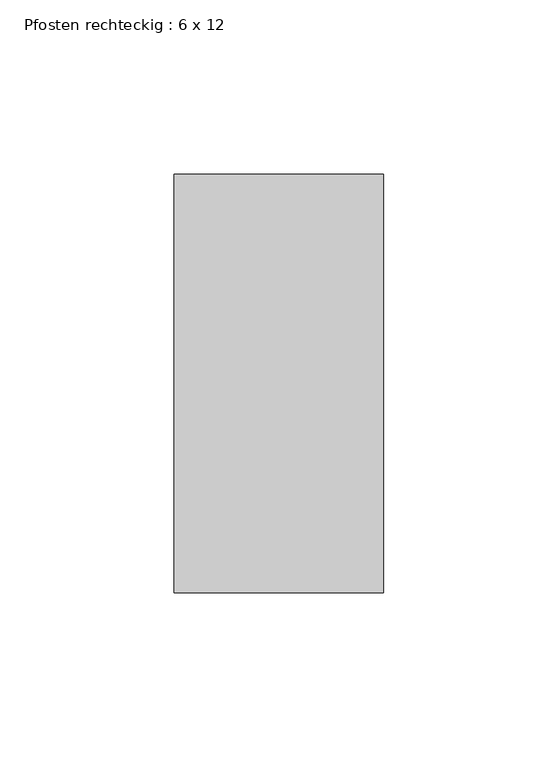
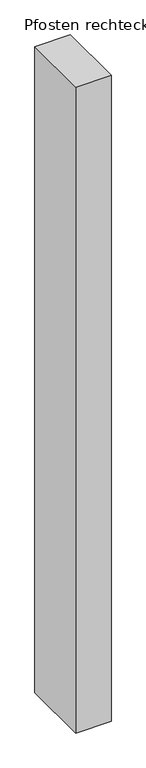
"""IFC4 building model written with IfcOpenShell, lengths in millimetres: member geometry, Pfosten rechteckig : 6 x 12."""

import ifcopenshell
import ifcopenshell.guid

model = None  # the IFC model being written
_history = None  # IfcOwnerHistory: only IFC2X3 demands one
_inside = {}  # id of a spatial element -> (the spatial element, [elements in it])
_under = {}  # id of a project, library or spatial element -> (it, [spatial elements below it])
_declared = {}  # id of a project -> (the project, [libraries it declares])
_typed = {}  # id of a type object -> (the type object, [elements of that type])
_made_of = {}  # id of a material, layer set ... -> (it, [elements and type objects made of it])


def new_model(schema):
    """Start an empty IFC model of exactly this schema.

    Asked for "IFC4X3", IfcOpenShell would pick the latest addendum, in which some entities
    have other attributes; the version numbers below select the first issue.
    IFC2X3 requires an IfcOwnerHistory on every rooted entity: one is made here for all.
    """
    global model, _history
    if schema == "IFC4X3":
        model = ifcopenshell.file(schema_version=(4, 3, 0, 0))
    else:
        model = ifcopenshell.file(schema=schema)
    _inside.clear()
    _under.clear()
    _declared.clear()
    _typed.clear()
    _made_of.clear()
    _history = None
    if model.schema == "IFC2X3":
        org = make("IfcOrganization", Name="unknown")
        user = make(
            "IfcPersonAndOrganization",
            ThePerson=make("IfcPerson", FamilyName="unknown"),
            TheOrganization=org,
        )
        app = make(
            "IfcApplication",
            ApplicationDeveloper=org,
            Version="unknown",
            ApplicationFullName="unknown",
            ApplicationIdentifier="unknown",
        )
        _history = make(
            "IfcOwnerHistory",
            OwningUser=user,
            OwningApplication=app,
            ChangeAction="ADDED",
            CreationDate=0,
        )
    return model


def make(cls, **values):
    """One entity of the class cls with the attributes given. An attribute that is None is left unset."""
    return model.create_entity(
        cls, **{name: value for name, value in values.items() if value is not None}
    )


def rooted(cls, **values):
    """An entity with a GlobalId (a new one), such as an element, a storey or a relation."""
    return make(cls, GlobalId=ifcopenshell.guid.new(), OwnerHistory=_history, **values)


def si_unit(unit_type, name, prefix=None):
    """IfcSIUnit, for example si_unit("LENGTHUNIT", "METRE", prefix="MILLI")."""
    return make("IfcSIUnit", UnitType=unit_type, Prefix=prefix, Name=name)


def assignment(units):
    """IfcUnitAssignment: the units of a project."""
    return None if units is None else make("IfcUnitAssignment", Units=units)


def point(xyz):
    """IfcCartesianPoint."""
    return None if xyz is None else make("IfcCartesianPoint", Coordinates=xyz)


def direction(xyz):
    """IfcDirection."""
    return None if xyz is None else make("IfcDirection", DirectionRatios=xyz)


def frame(location, z_axis=None, x_axis=None):
    """IfcAxis2Placement3D, a coordinate frame: its origin and axes. An axis left out is left unset."""
    return make(
        "IfcAxis2Placement3D",
        Location=point(location),
        Axis=direction(z_axis),
        RefDirection=direction(x_axis),
    )


def origin():
    """The frame at (0, 0, 0) with its axes left unset."""
    return frame((0.0, 0.0, 0.0))


def place(relative_to, where):
    """IfcLocalPlacement: puts the frame where relative to a parent placement (None: the world)."""
    return make(
        "IfcLocalPlacement", PlacementRelTo=relative_to, RelativePlacement=where
    )


def context(
    kind, dimensions, precision=None, world=None, true_north=None, identifier=None
):
    """IfcGeometricRepresentationContext, for example the 3D "Model" context."""
    return make(
        "IfcGeometricRepresentationContext",
        ContextIdentifier=identifier,
        ContextType=kind,
        CoordinateSpaceDimension=dimensions,
        Precision=precision,
        WorldCoordinateSystem=world,
        TrueNorth=true_north,
    )


def project(units=None, contexts=None):
    """IfcProject with its units and contexts."""
    return rooted(
        "IfcProject",
        Name="project",
        RepresentationContexts=contexts,
        UnitsInContext=assignment(units),
    )


def spatial(cls, under=None, at=None, **own):
    """A site, building, storey or space (cls), placed at a placement, below another one or the project."""
    s = rooted(cls, ObjectPlacement=at, **own)
    if under is not None:
        _under.setdefault(under.id(), (under, []))[1].append(s)
    return s


def polyline(points):
    """IfcPolyline through the points."""
    return make("IfcPolyline", Points=[point(p) for p in points])


def outline(outer, holes=None, kind="AREA"):
    """IfcArbitraryClosedProfileDef: a profile drawn as a closed curve; with holes, ...WithVoids."""
    if holes is None:
        return make("IfcArbitraryClosedProfileDef", ProfileType=kind, OuterCurve=outer)
    return make(
        "IfcArbitraryProfileDefWithVoids",
        ProfileType=kind,
        OuterCurve=outer,
        InnerCurves=holes,
    )


def extrude(swept, where, along, depth):
    """IfcExtrudedAreaSolid: the profile swept, set in the frame where, extruded along a direction by depth."""
    return make(
        "IfcExtrudedAreaSolid",
        SweptArea=swept,
        Position=where,
        ExtrudedDirection=direction(along),
        Depth=depth,
    )


def shape(context_of_items, identifier, shape_type, items):
    """IfcShapeRepresentation: the items that make up one representation, for example the "Body"."""
    return make(
        "IfcShapeRepresentation",
        ContextOfItems=context_of_items,
        RepresentationIdentifier=identifier,
        RepresentationType=shape_type,
        Items=items,
    )


def source(mapping_origin, context_of_items, identifier, shape_type, items):
    """IfcRepresentationMap: a shape defined once, which mapped items show again and again."""
    return make(
        "IfcRepresentationMap",
        MappingOrigin=mapping_origin,
        MappedRepresentation=shape(context_of_items, identifier, shape_type, items),
    )


def transform(
    local_origin,
    x_axis=None,
    y_axis=None,
    z_axis=None,
    scale=None,
    scale2=None,
    scale3=None,
    uniform=True,
):
    """IfcCartesianTransformationOperator3D, or its non-uniform kind. x_axis, y_axis, z_axis: its Axis1, 2, 3."""
    if uniform:
        return make(
            "IfcCartesianTransformationOperator3D",
            Axis1=direction(x_axis),
            Axis2=direction(y_axis),
            LocalOrigin=point(local_origin),
            Scale=scale,
            Axis3=direction(z_axis),
        )
    return make(
        "IfcCartesianTransformationOperator3DnonUniform",
        Axis1=direction(x_axis),
        Axis2=direction(y_axis),
        LocalOrigin=point(local_origin),
        Scale=scale,
        Axis3=direction(z_axis),
        Scale2=scale2,
        Scale3=scale3,
    )


def mapped(mapping_source, mapping_target):
    """IfcMappedItem: shows the shape of a source again, moved by a transform."""
    return make(
        "IfcMappedItem", MappingSource=mapping_source, MappingTarget=mapping_target
    )


def made_of(thing, what):
    """Note that an element or type object is made of a material, layer set ...; save() writes the relation."""
    if what is not None:
        _made_of.setdefault(what.id(), (what, []))[1].append(thing)
    return thing


def element(
    cls,
    number,
    at=None,
    inside=None,
    cuts=None,
    type_object=None,
    material=None,
    context=None,
    identifier="Body",
    shape_type=None,
    held_by="IfcProductDefinitionShape",
    body=None,
    shapes=None,
    **own,
):
    """One element of the class cls, such as IfcWall. Its Tag is "e" and its number.

    at: its placement. inside: the storey or other place that contains it. cuts: it is an
    opening in that element (IfcRelVoidsElement). A single representation is given by context,
    identifier, shape_type and body (its items); several are given by shapes. held_by: the class
    of the entity that holds the representations. save() writes the other relations.
    """
    e = rooted(cls, Tag="e%d" % number, ObjectPlacement=at, **own)
    if body is not None:
        shapes = [shape(context, identifier, shape_type, body)]
    if shapes is not None:
        e.Representation = make(held_by, Representations=shapes)
    if inside is not None:
        _inside.setdefault(inside.id(), (inside, []))[1].append(e)
    if cuts is not None:
        rooted(
            "IfcRelVoidsElement", RelatingBuildingElement=cuts, RelatedOpeningElement=e
        )
    if type_object is not None:
        _typed.setdefault(type_object.id(), (type_object, []))[1].append(e)
    return made_of(e, material)


def aggregate(whole, parts):
    """IfcRelAggregates: a whole, such as a stair, and the parts it consists of."""
    return rooted("IfcRelAggregates", RelatingObject=whole, RelatedObjects=parts)


def save(model, path):
    """Write the relations noted so far, then the file.

    IfcRelAggregates (storeys below a building ...), IfcRelContainedInSpatialStructure (elements
    in a storey), IfcRelDefinesByType, IfcRelAssociatesMaterial and IfcRelDeclares: one each for
    every whole, place, type object, material and project.
    """
    for whole, parts in _under.values():
        aggregate(whole, parts)
    for where, things in _inside.values():
        rooted(
            "IfcRelContainedInSpatialStructure",
            RelatedElements=things,
            RelatingStructure=where,
        )
    for kind, things in _typed.values():
        rooted("IfcRelDefinesByType", RelatedObjects=things, RelatingType=kind)
    for what, things in _made_of.values():
        rooted("IfcRelAssociatesMaterial", RelatedObjects=things, RelatingMaterial=what)
    for by, libraries in _declared.values():
        rooted("IfcRelDeclares", RelatingContext=by, RelatedDefinitions=libraries)
    model.write(path)


def pfosten_rechteckig_6_x_12_ce3c1f4b(model_context):
    return source(origin(), model_context, "Body", "SweptSolid", [
        extrude(outline(polyline([(30.0, 60.0), (30.0, -60.0), (-30.0, -60.0), (-30.0, 60.0), (30.0, 60.0)])), frame((0.0, 0.0, -1160.0000003), z_axis=(0.0, 0.0, 1.0), x_axis=(1.0, 0.0, 0.0)), (0.0, 0.0, 1.0), 1160.0000003),
    ])


if __name__ == "__main__":
    model = new_model("IFC4")
    model_context = context("Model", 3, world=origin())
    ifc_project = project(units=[si_unit("LENGTHUNIT", "METRE", prefix="MILLI")], contexts=[model_context])
    site = spatial("IfcSite", under=ifc_project)
    building = spatial("IfcBuilding", under=site)
    placement = place(None, origin())
    pfosten_rechteckig_6_x_12_shape = pfosten_rechteckig_6_x_12_ce3c1f4b(model_context)
    element("IfcMember", 1, ObjectType="Pfosten rechteckig : 6 x 12", at=placement, inside=building, context=model_context, shape_type="MappedRepresentation", body=[
        mapped(pfosten_rechteckig_6_x_12_shape, transform((0.0, 0.0, 0.0), x_axis=(1.0, 0.0, 0.0), y_axis=(0.0, 1.0, 0.0), z_axis=(0.0, 0.0, 1.0))),
    ])
    save(model, "model.ifc")

# Revit data of these elements
# Type "Pfosten rechteckig : 6 x 12"
#   built-in parameter 1007304 = 0.393701 (stored number, unit not read)
#   built-in parameter 1007301 = 0.0984252 (stored number, unit not read)
#   built-in parameter 1007300 = 0.0984252 (stored number, unit not read)
# Element 1 (IfcMember, "Pfosten rechteckig : 6 x 12")
#   Materials on its faces: "Metall - verzinkt"
# Materials
#   "Metall - verzinkt": class "Allgemeines", colour RGB 200 200 200, transparency 0, Cost = 0
